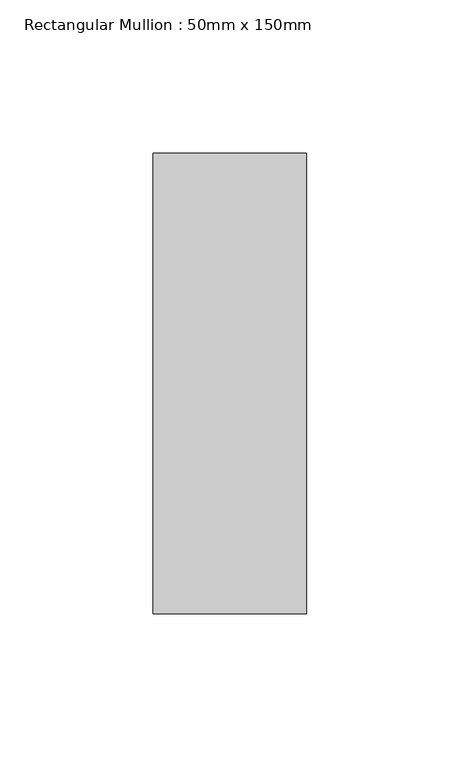
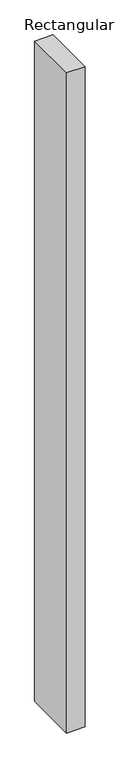
"""IFC4 building model written with IfcOpenShell, lengths in millimetres: member geometry, Rectangular Mullion : 50mm x 150mm."""

from ifc_helpers import new_model, si_unit, frame, origin, place, context, project, spatial, polyline, outline, extrude, source, transform, mapped, element, save


def rectangular_mullion_50mm_x_150mm_0c966fbd(model_context):
    return source(origin(), model_context, "Body", "SweptSolid", [
        extrude(outline(polyline([(0.0, 75.0), (0.0, -75.0), (-50.0, -75.0), (-50.0, 75.0), (0.0, 75.0)])), frame((0.0, 0.0, -1887.3779433), z_axis=(0.0, 0.0, 1.0), x_axis=(1.0, 0.0, 0.0)), (0.0, 0.0, 1.0), 1887.3779433),
    ])


if __name__ == "__main__":
    model = new_model("IFC4")
    model_context = context("Model", 3, world=origin())
    ifc_project = project(units=[si_unit("LENGTHUNIT", "METRE", prefix="MILLI")], contexts=[model_context])
    site = spatial("IfcSite", under=ifc_project)
    building = spatial("IfcBuilding", under=site)
    placement = place(None, origin())
    rectangular_mullion_50mm_x_150mm_shape = rectangular_mullion_50mm_x_150mm_0c966fbd(model_context)
    element("IfcMember", 1, ObjectType="Rectangular Mullion : 50mm x 150mm", at=placement, inside=building, context=model_context, shape_type="MappedRepresentation", body=[
        mapped(rectangular_mullion_50mm_x_150mm_shape, transform((0.0, 0.0, 0.0), x_axis=(1.0, 0.0, 0.0), y_axis=(0.0, 1.0, 0.0), z_axis=(0.0, 0.0, 1.0))),
    ])
    save(model, "model.ifc")

# Revit data of these elements
# Type "Rectangular Mullion : 50mm x 150mm"
#   built-in parameter 1007304 = 0.492126 (stored number, unit not read)
#   built-in parameter 1007301 = 0.082021 (stored number, unit not read)
#   built-in parameter 1007300 = 0.082021 (stored number, unit not read)
# Element 1 (IfcMember, "Rectangular Mullion : 50mm x 150mm")
#   Materials on its faces: "Aluminum"
# Materials
#   "Aluminum": class "Metal", colour RGB 244 244 244, transparency 0, Description = "Aluminum 6061", Cost = 0
